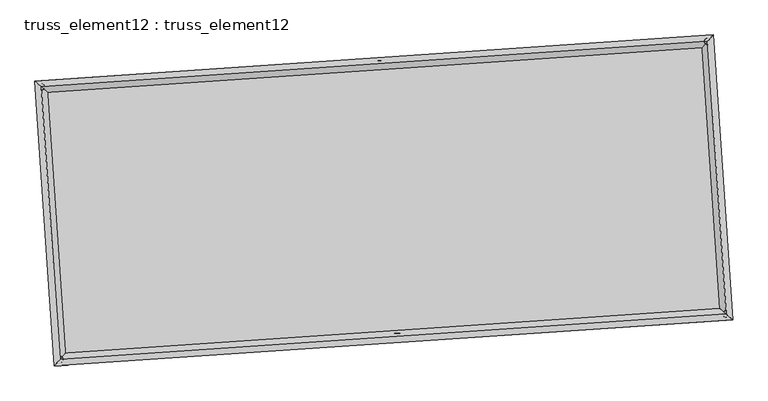
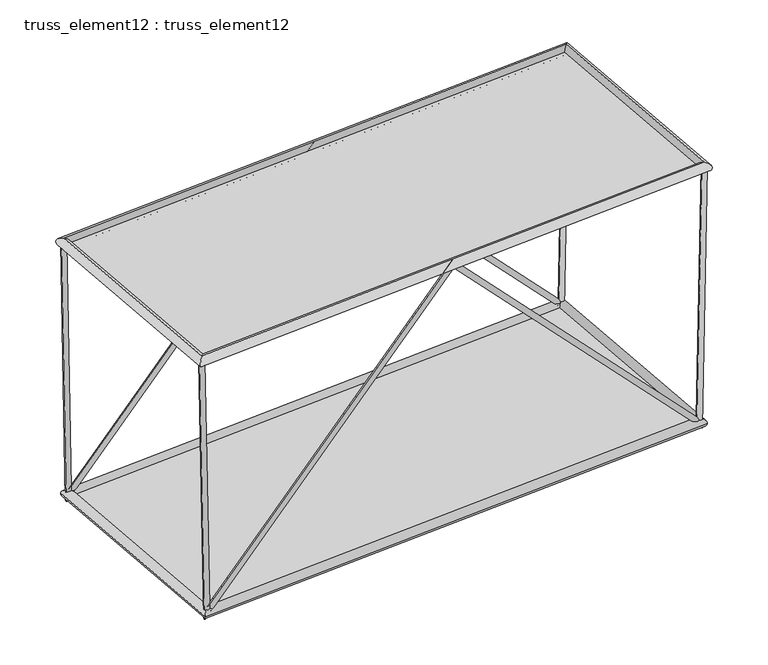
"""IFC4 building model written with IfcOpenShell, lengths in millimetres: plate geometry, truss_element12 : truss_element12."""

from ifc_helpers import new_model, si_unit, frame, origin, origin_with_axes, place, context, project, spatial, polyline, circle_curve, ellipse_curve, outline, extrude, source, transform, mapped, element, save
from ifc_brep_helpers import plane_surface, cylinder_surface, advanced_brep


def truss_element12_truss_element12_8118c823(model_context):
    return source(origin(), model_context, "Body", "SolidModel", [
        advanced_brep(
        [(-3759.0101005, 2269.8097873, 5000.0518193), (-3858.0957712, 2256.449774, 4998.1703582), (-3667.2244266, 2276.0683035, 121.7906411), (-3761.7624562, 2263.0183766, -121.7906411), (1064.425668, 2598.7015368, 5071.2149108), (1064.8633229, 2592.1276407, 4926.9805686), (5794.6969904, 2921.2407568, 121.7809717), (5890.0639866, 2921.1397317, -121.7809717), (5887.8511571, 2927.5925853, 5000.0391427), (5987.8326962, 2927.8062083, 4998.1296386)],
        [
            (0, 1, circle_curve(frame((-3808.5529358, 2263.1297807, 4999.1110888), z_axis=(-0.018811898886610594, -0.001282711874355422, 0.9998222177519999), x_axis=(-0.13360051524293703, 0.9910344893322439, -0.0012422885334351164)), 50.0)),
            (1, 0, circle_curve(frame((-3808.5529358, 2263.1297807, 4999.1110888), z_axis=(-0.018811898886610594, -0.001282711874355422, 0.9998222177519999), x_axis=(-0.13360051524293703, 0.9910344893322439, -0.0012422885334351164)), 50.0)),
            (0, 2),
            (2, 3, ellipse_curve(frame((-3714.4934414, 2269.54334, 0.0), z_axis=(-0.9292247210951419, -0.06336030141761893, 0.3640424287221536), x_axis=(0.3631990866028644, 0.024765165066465387, 0.9313823651380112)), 131.0480431, 50.0)),
            (3, 1),
            (3, 2, ellipse_curve(frame((-3714.4934414, 2269.54334, 0.0), z_axis=(-0.9292247210951419, -0.06336030141761893, 0.3640424287221536), x_axis=(0.3631990866028644, 0.024765165066465387, 0.9313823651380112)), 131.0480431, 50.0)),
            (2, 4),
            (4, 5, ellipse_curve(frame((1064.6444954, 2595.4145888, 4999.0977397), z_axis=(-0.9976833933961031, -0.06802823804604483, 7.328019523198135e-05), x_axis=(-7.311043404423826e-05, -4.985122578868747e-06, -0.9999999973150066)), 72.2742041, 50.0)),
            (5, 3),
            (5, 4, ellipse_curve(frame((1064.6444954, 2595.4145888, 4999.0977397), z_axis=(-0.9976833933961031, -0.06802823804604483, 7.328019523198135e-05), x_axis=(-7.311043404423826e-05, -4.985122578868747e-06, -0.9999999973150066)), 72.2742041, 50.0)),
            (4, 6),
            (6, 7, ellipse_curve(frame((5842.3804885, 2921.1902443, 0.0), z_axis=(-0.9293023610631934, -0.06336559539190303, -0.3638432671398546), x_axis=(-0.3630003863990688, -0.024751616454898564, 0.9314601853847518)), 131.026691, 50.0)),
            (7, 5),
            (7, 6, ellipse_curve(frame((5842.3804885, 2921.1902443, 0.0), z_axis=(-0.9293023610631934, -0.06336559539190303, -0.3638432671398546), x_axis=(-0.3630003863990688, -0.024751616454898564, 0.9314601853847518)), 131.026691, 50.0)),
            (8, 9, circle_curve(frame((5937.8419267, 2927.6993968, 4999.0843906), z_axis=(0.019092287634230168, 0.001301830517198297, 0.9998168781282882), x_axis=(-0.002160697205567338, 0.9999968708746868, -0.0012608046719796988)), 50.0)),
            (9, 8, circle_curve(frame((5937.8419267, 2927.6993968, 4999.0843906), z_axis=(0.019092287634230168, 0.001301830517198297, 0.9998168781282882), x_axis=(-0.002160697205567338, 0.9999968708746868, -0.0012608046719796988)), 50.0)),
            (6, 8),
            (9, 7),
        ],
        [
            plane_surface(frame((-3808.5529358, 2313.1297395, 4999.1752357), z_axis=(-0.0188118988866116, -0.0012827118743585508, 0.9998222177519999), x_axis=(0.9998230405728206, -2.41345169111895e-05, 0.01881188340504991))),
            cylinder_surface(frame((-3808.5529358, 2263.1297807, 4999.1110888), z_axis=(-0.018811898886610594, -0.001282711874355422, 0.9998222177519999), x_axis=(-0.13360051524293703, 0.9910344893322439, -0.0012422885334351164)), 50.0),
            cylinder_surface(frame((-3714.4934414, 2269.54334, 0.0), z_axis=(-0.6902599032026427, -0.04706619887584547, -0.7220291122621425), x_axis=(-0.02042017886587182, 0.9987518262310586, -0.04558295619210198)), 50.0),
            cylinder_surface(frame((1064.6444954, 2595.4145888, 4999.0977397), z_axis=(-0.690154320065973, -0.04705899956311478, 0.7221305041710904), x_axis=(-0.11534734726939705, 0.9922791034695722, -0.04557598375828237)), 50.0),
            plane_surface(frame((5937.8419267, 2877.6994392, 4999.149494), z_axis=(0.019092287634229446, 0.0013018305172036945, 0.9998168781282883), x_axis=(0.9998177256644792, -2.485945392649572e-05, -0.01909227144987471))),
            cylinder_surface(frame((5842.3804885, 2921.1902443, 0.0), z_axis=(-0.019092287634230168, -0.001301830517198297, -0.9998168781282882), x_axis=(-0.002160697205567338, 0.9999968708746868, -0.0012608046719796988)), 50.0),
        ],
        [
            (0, [[1, 2]]),
            (1, [[-1, 3, 4, 5]]),
            (1, [[-2, -5, 6, -3]]),
            (2, [[-4, 7, 8, 9]]),
            (2, [[-6, -9, 10, -7]]),
            (3, [[-8, 11, 12, 13]]),
            (3, [[-10, -13, 14, -11]]),
            (4, [[15, 16]]),
            (5, [[-12, 17, -16, 18]]),
            (5, [[-14, -18, -15, -17]]),
        ],
    ),
        advanced_brep(
        [(-3486.8971476, -1720.923797, 5000.0518193), (-3585.9828183, -1734.2838103, 4998.1703582), (-3395.1114737, -1714.6652808, 121.7906411), (-3489.6495033, -1727.7152077, -121.7906411), (1336.5386209, -1392.0320475, 5071.2149108), (1336.9762758, -1398.6059436, 4926.9805686), (6066.8099433, -1069.4928275, 121.7809717), (6162.1769395, -1069.5938526, -121.7809717), (6159.96411, -1063.140999, 5000.0391427), (6259.9456491, -1062.927376, 4998.1296386)],
        [
            (0, 1, circle_curve(frame((-3536.4399829, -1727.6038036, 4999.1110888), z_axis=(-0.018811898886610712, -0.0012827118743554558, 0.999822217752), x_axis=(-0.13360051524293726, 0.9910344893322439, -0.0012422885334351028)), 50.0)),
            (1, 0, circle_curve(frame((-3536.4399829, -1727.6038036, 4999.1110888), z_axis=(-0.018811898886610712, -0.0012827118743554558, 0.999822217752), x_axis=(-0.13360051524293726, 0.9910344893322439, -0.0012422885334351028)), 50.0)),
            (0, 2),
            (2, 3, ellipse_curve(frame((-3442.3804885, -1721.1902443, 0.0), z_axis=(-0.9292247210951418, -0.0633603014176191, 0.3640424287221536), x_axis=(0.3631990866028643, 0.02476516506646543, 0.9313823651380113)), 131.0480431, 50.0)),
            (3, 1),
            (3, 2, ellipse_curve(frame((-3442.3804885, -1721.1902443, 0.0), z_axis=(-0.9292247210951418, -0.0633603014176191, 0.3640424287221536), x_axis=(0.3631990866028643, 0.02476516506646543, 0.9313823651380113)), 131.0480431, 50.0)),
            (2, 4),
            (4, 5, ellipse_curve(frame((1336.7574483, -1395.3189955, 4999.0977397), z_axis=(-0.9976833933961031, -0.06802823804604513, 7.328019523166036e-05), x_axis=(-7.311043404393078e-05, -4.985122578705386e-06, -0.9999999973150066)), 72.2742041, 50.0)),
            (5, 3),
            (5, 4, ellipse_curve(frame((1336.7574483, -1395.3189955, 4999.0977397), z_axis=(-0.9976833933961031, -0.06802823804604513, 7.328019523166036e-05), x_axis=(-7.311043404393078e-05, -4.985122578705386e-06, -0.9999999973150066)), 72.2742041, 50.0)),
            (4, 6),
            (6, 7, ellipse_curve(frame((6114.4934414, -1069.54334, 0.0), z_axis=(-0.9293023610631932, -0.06336559539190349, -0.36384326713985504), x_axis=(-0.36300038639906934, -0.024751616454898748, 0.9314601853847516)), 131.026691, 50.0)),
            (7, 5),
            (7, 6, ellipse_curve(frame((6114.4934414, -1069.54334, 0.0), z_axis=(-0.9293023610631932, -0.06336559539190349, -0.36384326713985504), x_axis=(-0.36300038639906934, -0.024751616454898748, 0.9314601853847516)), 131.026691, 50.0)),
            (8, 9, circle_curve(frame((6209.9548796, -1063.0341875, 4999.0843906), z_axis=(0.019092287634229887, 0.0013018305171983192, 0.9998168781282882), x_axis=(-0.002160697205567476, 0.9999968708746868, -0.0012608046719797192)), 50.0)),
            (9, 8, circle_curve(frame((6209.9548796, -1063.0341875, 4999.0843906), z_axis=(0.019092287634229887, 0.0013018305171983192, 0.9998168781282882), x_axis=(-0.002160697205567476, 0.9999968708746868, -0.0012608046719797192)), 50.0)),
            (6, 8),
            (9, 7),
        ],
        [
            plane_surface(frame((-3536.4399829, -1677.6038448, 4999.1752357), z_axis=(-0.0188118988866116, -0.0012827118743585543, 0.9998222177519999), x_axis=(0.9998230405728206, -2.41345169111895e-05, 0.01881188340504991))),
            cylinder_surface(frame((-3536.4399829, -1727.6038036, 4999.1110888), z_axis=(-0.01881189888661071, -0.0012827118743554556, 0.9998222177519998), x_axis=(-0.13360051524293726, 0.9910344893322439, -0.0012422885334351028)), 50.0),
            cylinder_surface(frame((-3442.3804885, -1721.1902443, 0.0), z_axis=(-0.6902599032026429, -0.04706619887584558, -0.7220291122621424), x_axis=(-0.020420178865871896, 0.9987518262310586, -0.045582956192102064)), 50.0),
            cylinder_surface(frame((1336.7574483, -1395.3189955, 4999.0977397), z_axis=(-0.6901543200659735, -0.04705899956311514, 0.72213050417109), x_axis=(-0.11534734726939751, 0.9922791034695722, -0.04557598375828241)), 50.0),
            plane_surface(frame((6209.9548796, -1113.0341451, 4999.149494), z_axis=(0.019092287634229446, 0.001301830517192873, 0.9998168781282883), x_axis=(0.9998177256644792, -2.485945392560754e-05, -0.01909227144987471))),
            cylinder_surface(frame((6114.4934414, -1069.54334, 0.0), z_axis=(-0.019092287634229887, -0.0013018305171983192, -0.9998168781282882), x_axis=(-0.002160697205567476, 0.9999968708746868, -0.0012608046719797192)), 50.0),
        ],
        [
            (0, [[1, 2]]),
            (1, [[-1, 3, 4, 5]]),
            (1, [[-2, -5, 6, -3]]),
            (2, [[-4, 7, 8, 9]]),
            (2, [[-6, -9, 10, -7]]),
            (3, [[-8, 11, 12, 13]]),
            (3, [[-10, -13, 14, -11]]),
            (4, [[15, 16]]),
            (5, [[-12, 17, -16, 18]]),
            (5, [[-14, -18, -15, -17]]),
        ],
    ),
        advanced_brep(
        [(-3536.4469431, -1727.6115178, 4909.1110891), (-3536.4330228, -1727.5960894, 5089.1110885), (-3808.544993, 2263.1230826, 5089.1110885), (-3808.5608787, 2263.1364787, 4909.1110891), (5937.8354573, 2927.6917161, 5089.0843904), (5937.848396, 2927.7070776, 4909.0843909), (6209.9474275, -1063.027456, 5089.0843904), (6209.9623317, -1063.040919, 4909.0843909)],
        [
            (0, 1, ellipse_curve(frame((-3536.4399829, -1727.6038036, 4999.1110888), z_axis=(-0.7535719234028208, 0.6573654662782634, 1.932477302402373e-06), x_axis=(-0.6573654662754491, -0.7535719234052757, 1.932477302785358e-06)), 127.2792206, 90.0)),
            (1, 2),
            (2, 3, ellipse_curve(frame((-3808.5529358, 2263.1297807, 4999.1110888), z_axis=(-0.6573654662754492, -0.7535719234052756, 1.93247730270711e-06), x_axis=(0.7535719234028205, -0.6573654662782638, -1.9324773023241237e-06)), 127.2792206, 90.0)),
            (3, 0),
            (1, 0, ellipse_curve(frame((-3536.4399829, -1727.6038036, 4999.1110888), z_axis=(-0.7535719234028208, 0.6573654662782634, 1.932477302402373e-06), x_axis=(-0.6573654662754491, -0.7535719234052757, 1.932477302785358e-06)), 127.2792206, 90.0)),
            (3, 2, ellipse_curve(frame((-3808.5529358, 2263.1297807, 4999.1110888), z_axis=(-0.6573654662754492, -0.7535719234052756, 1.93247730270711e-06), x_axis=(0.7535719234028205, -0.6573654662782638, -1.9324773023241237e-06)), 127.2792206, 90.0)),
            (2, 4),
            (4, 5, ellipse_curve(frame((5937.8419267, 2927.6993968, 4999.0843906), z_axis=(-0.7535719234028213, 0.6573654662782629, 1.932477302515678e-06), x_axis=(-0.6573654662754486, -0.7535719234052763, 1.932477302515556e-06)), 127.2792206, 90.0)),
            (5, 3),
            (5, 4, ellipse_curve(frame((5937.8419267, 2927.6993968, 4999.0843906), z_axis=(-0.7535719234028213, 0.6573654662782629, 1.932477302515678e-06), x_axis=(-0.6573654662754486, -0.7535719234052763, 1.932477302515556e-06)), 127.2792206, 90.0)),
            (4, 6),
            (6, 7, ellipse_curve(frame((6209.9548796, -1063.0341875, 4999.0843906), z_axis=(0.6573654662754486, 0.7535719234052763, -1.932477302593805e-06), x_axis=(-0.7535719234028213, 0.6573654662782628, 1.932477302593927e-06)), 127.2792206, 90.0)),
            (7, 5),
            (7, 6, ellipse_curve(frame((6209.9548796, -1063.0341875, 4999.0843906), z_axis=(0.6573654662754486, 0.7535719234052763, -1.932477302593805e-06), x_axis=(-0.7535719234028213, 0.6573654662782628, 1.932477302593927e-06)), 127.2792206, 90.0)),
            (6, 1),
            (0, 7),
        ],
        [
            cylinder_surface(frame((-3536.4399829, -1727.6038036, 4999.1110888), z_axis=(0.06802823822869636, -0.997683396074877, 0.0), x_axis=(-0.997683392639436, -0.0680282379944467, 8.298696282030801e-05)), 90.0),
            cylinder_surface(frame((-3808.5529358, 2263.1297807, 4999.1110888), z_axis=(-0.997683396071151, -0.06802823822844395, 2.7329356101957602e-06), x_axis=(-0.06802823779080196, 0.9976833928769032, 8.025402721864263e-05)), 90.0),
            cylinder_surface(frame((5937.8419267, 2927.6993968, 4999.0843906), z_axis=(-0.06802823822869826, 0.997683396074877, 0.0), x_axis=(0.9976833930770779, 0.06802823802428974, 7.752109161724803e-05)), 90.0),
            cylinder_surface(frame((6209.9548796, -1063.0341875, 4999.0843906), z_axis=(0.997683396071151, 0.06802823822844414, -2.7329356103064204e-06), x_axis=(0.06802823822844414, -0.9976833928470621, 8.025402721875352e-05)), 90.0),
        ],
        [
            (0, [[1, 2, 3, 4]]),
            (0, [[5, -4, 6, -2]]),
            (1, [[-3, 7, 8, 9]]),
            (1, [[-6, -9, 10, -7]]),
            (2, [[-8, 11, 12, 13]]),
            (2, [[-10, -13, 14, -11]]),
            (3, [[-12, 15, -1, 16]]),
            (3, [[-14, -16, -5, -15]]),
        ],
    ),
        advanced_brep(
        [(-3358.7115243, -1625.2761972, 0.0), (-3526.0494527, -1817.1042913, 0.0), (-3810.4074885, 2353.2123043, 0.0), (-3618.5793943, 2185.8743758, 0.0), (5926.0494527, 3017.1042913, 0.0), (5758.7115243, 2825.2761972, 0.0), (6210.4074885, -1153.2123043, 0.0), (6018.5793943, -985.8743758, 0.0)],
        [
            (0, 1, ellipse_curve(frame((-3442.3804885, -1721.1902443, 0.0), z_axis=(-0.7535719234054569, 0.6573654662780819, 0.0), x_axis=(-0.6573654662780818, -0.7535719234054571, 0.0)), 127.2792206, 90.0)),
            (1, 2),
            (2, 3, ellipse_curve(frame((-3714.4934414, 2269.54334, 0.0), z_axis=(-0.6573654662780819, -0.753571923405457, 0.0), x_axis=(0.7535719234054569, -0.6573654662780819, 0.0)), 127.2792206, 90.0)),
            (3, 0),
            (1, 0, ellipse_curve(frame((-3442.3804885, -1721.1902443, 0.0), z_axis=(-0.7535719234054569, 0.6573654662780819, 0.0), x_axis=(-0.6573654662780818, -0.7535719234054571, 0.0)), 127.2792206, 90.0)),
            (3, 2, ellipse_curve(frame((-3714.4934414, 2269.54334, 0.0), z_axis=(-0.6573654662780819, -0.753571923405457, 0.0), x_axis=(0.7535719234054569, -0.6573654662780819, 0.0)), 127.2792206, 90.0)),
            (2, 4),
            (4, 5, ellipse_curve(frame((5842.3804885, 2921.1902443, 0.0), z_axis=(-0.7535719234054578, 0.657365466278081, 0.0), x_axis=(-0.657365466278081, -0.7535719234054576, 0.0)), 127.2792206, 90.0)),
            (5, 3),
            (5, 4, ellipse_curve(frame((5842.3804885, 2921.1902443, 0.0), z_axis=(-0.7535719234054578, 0.657365466278081, 0.0), x_axis=(-0.657365466278081, -0.7535719234054576, 0.0)), 127.2792206, 90.0)),
            (4, 6),
            (6, 7, ellipse_curve(frame((6114.4934414, -1069.54334, 0.0), z_axis=(0.6573654662780811, 0.7535719234054576, 0.0), x_axis=(-0.7535719234054576, 0.6573654662780812, 0.0)), 127.2792206, 90.0)),
            (7, 5),
            (7, 6, ellipse_curve(frame((6114.4934414, -1069.54334, 0.0), z_axis=(0.6573654662780811, 0.7535719234054576, 0.0), x_axis=(-0.7535719234054576, 0.6573654662780812, 0.0)), 127.2792206, 90.0)),
            (6, 1),
            (0, 7),
        ],
        [
            cylinder_surface(frame((-3442.3804885, -1721.1902443, 0.0), z_axis=(0.06802823822869888, -0.9976833960748768, 0.0), x_axis=(-0.9976833960748768, -0.06802823822869888, 0.0)), 90.0),
            cylinder_surface(frame((-3714.4934414, 2269.54334, 0.0), z_axis=(-0.9976833960748767, -0.06802823822870076, 0.0), x_axis=(-0.06802823822870076, 0.9976833960748767, 0.0)), 90.0),
            cylinder_surface(frame((5842.3804885, 2921.1902443, 0.0), z_axis=(-0.06802823822870105, 0.9976833960748767, 0.0), x_axis=(0.9976833960748767, 0.06802823822870105, 0.0)), 90.0),
            cylinder_surface(frame((6114.4934414, -1069.54334, 0.0), z_axis=(0.9976833960748767, 0.06802823822870052, 0.0), x_axis=(0.06802823822870052, -0.9976833960748767, 0.0)), 90.0),
        ],
        [
            (0, [[1, 2, 3, 4]]),
            (0, [[5, -4, 6, -2]]),
            (1, [[-3, 7, 8, 9]]),
            (1, [[-6, -9, 10, -7]]),
            (2, [[-8, 11, 12, 13]]),
            (2, [[-10, -13, 14, -11]]),
            (3, [[-12, 15, -1, 16]]),
            (3, [[-14, -16, -5, -15]]),
        ],
    ),
        extrude(outline(polyline([(-3442.3804885, -1721.1902443), (-3714.4934414, 2269.54334), (5842.3804885, 2921.1902443), (6114.4934414, -1069.54334), (-3442.3804885, -1721.1902443)])), origin_with_axes(), (0.0, 0.0, 1.0), 20.0),
        extrude(outline(polyline([(-2000.0, 4884.5129131), (2000.0, 4884.512913), (2000.0, -4884.5129131), (-2000.0, -4884.512913), (-2000.0, 4884.5129131)])), frame((1200.7009719, 600.0477966, 4999.0977397), z_axis=(2.726604480815564e-06, 1.8591679502417433e-07, 0.9999999999962655), x_axis=(-0.06802823822869859, 0.9976833960748768, 0.0)), (0.0, 0.0, 1.0), 20.0),
    ])


if __name__ == "__main__":
    model = new_model("IFC4")
    model_context = context("Model", 3, world=origin())
    ifc_project = project(units=[si_unit("LENGTHUNIT", "METRE", prefix="MILLI")], contexts=[model_context])
    site = spatial("IfcSite", under=ifc_project)
    building = spatial("IfcBuilding", under=site)
    placement = place(None, origin())
    truss_element12_truss_element12_shape = truss_element12_truss_element12_8118c823(model_context)
    element("IfcPlate", 1, ObjectType="truss_element12 : truss_element12", at=placement, inside=building, context=model_context, shape_type="MappedRepresentation", body=[
        mapped(truss_element12_truss_element12_shape, transform((0.0, 0.0, 0.0), x_axis=(1.0, 0.0, 0.0), y_axis=(0.0, 1.0, 0.0), z_axis=(0.0, 0.0, 1.0))),
    ])
    save(model, "model.ifc")

# Revit data of these elements
# Type "truss_element12 : truss_element12"
#   steellbar1 = 90 mm
#   steelbar2 = 50 mm
#   offset1 = 5000 mm
#   M = Default Roof
# Element 1 (IfcPlate, "truss_element12 : truss_element12")
#   Materials on its faces: "Default Roof"
# Materials
#   "Default Roof": class "Miscellaneous", colour RGB 0 127 0, transparency 0, Comments = "Rendering appearance not upgraded Rendering appearance not upgraded ", Cost = 0
